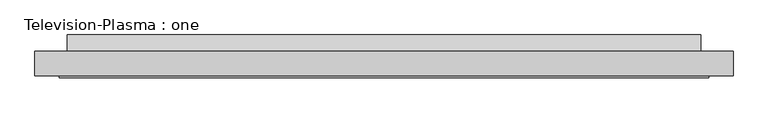
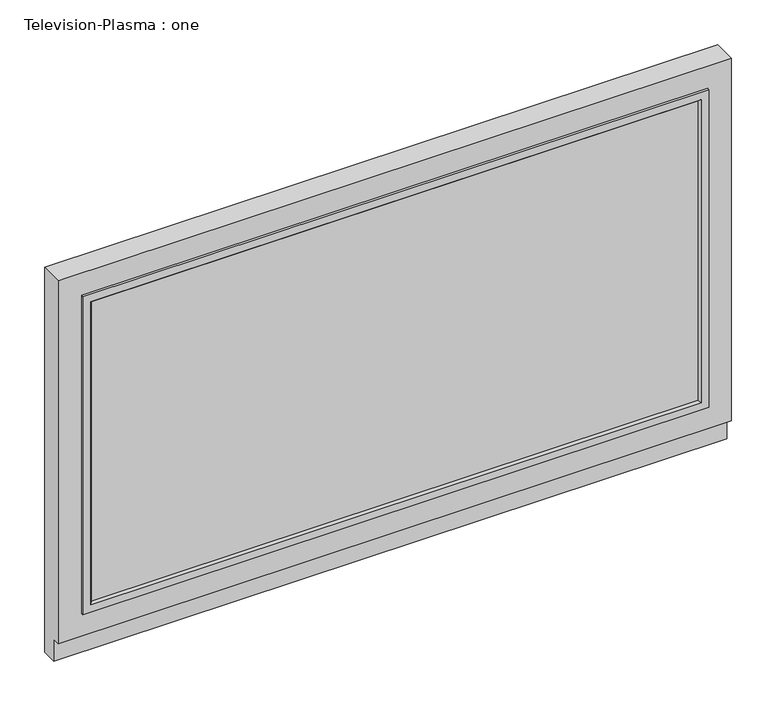
"""IFC4 building model written with IfcOpenShell, lengths in millimetres: furniture geometry, Television-Plasma : one."""

import ifcopenshell
import ifcopenshell.guid

model = None  # the IFC model being written
_history = None  # IfcOwnerHistory: only IFC2X3 demands one
_inside = {}  # id of a spatial element -> (the spatial element, [elements in it])
_under = {}  # id of a project, library or spatial element -> (it, [spatial elements below it])
_declared = {}  # id of a project -> (the project, [libraries it declares])
_typed = {}  # id of a type object -> (the type object, [elements of that type])
_made_of = {}  # id of a material, layer set ... -> (it, [elements and type objects made of it])


def new_model(schema):
    """Start an empty IFC model of exactly this schema.

    Asked for "IFC4X3", IfcOpenShell would pick the latest addendum, in which some entities
    have other attributes; the version numbers below select the first issue.
    IFC2X3 requires an IfcOwnerHistory on every rooted entity: one is made here for all.
    """
    global model, _history
    if schema == "IFC4X3":
        model = ifcopenshell.file(schema_version=(4, 3, 0, 0))
    else:
        model = ifcopenshell.file(schema=schema)
    _inside.clear()
    _under.clear()
    _declared.clear()
    _typed.clear()
    _made_of.clear()
    _history = None
    if model.schema == "IFC2X3":
        org = make("IfcOrganization", Name="unknown")
        user = make(
            "IfcPersonAndOrganization",
            ThePerson=make("IfcPerson", FamilyName="unknown"),
            TheOrganization=org,
        )
        app = make(
            "IfcApplication",
            ApplicationDeveloper=org,
            Version="unknown",
            ApplicationFullName="unknown",
            ApplicationIdentifier="unknown",
        )
        _history = make(
            "IfcOwnerHistory",
            OwningUser=user,
            OwningApplication=app,
            ChangeAction="ADDED",
            CreationDate=0,
        )
    return model


def make(cls, **values):
    """One entity of the class cls with the attributes given. An attribute that is None is left unset."""
    return model.create_entity(
        cls, **{name: value for name, value in values.items() if value is not None}
    )


def rooted(cls, **values):
    """An entity with a GlobalId (a new one), such as an element, a storey or a relation."""
    return make(cls, GlobalId=ifcopenshell.guid.new(), OwnerHistory=_history, **values)


def si_unit(unit_type, name, prefix=None):
    """IfcSIUnit, for example si_unit("LENGTHUNIT", "METRE", prefix="MILLI")."""
    return make("IfcSIUnit", UnitType=unit_type, Prefix=prefix, Name=name)


def assignment(units):
    """IfcUnitAssignment: the units of a project."""
    return None if units is None else make("IfcUnitAssignment", Units=units)


def point(xyz):
    """IfcCartesianPoint."""
    return None if xyz is None else make("IfcCartesianPoint", Coordinates=xyz)


def direction(xyz):
    """IfcDirection."""
    return None if xyz is None else make("IfcDirection", DirectionRatios=xyz)


def frame(location, z_axis=None, x_axis=None):
    """IfcAxis2Placement3D, a coordinate frame: its origin and axes. An axis left out is left unset."""
    return make(
        "IfcAxis2Placement3D",
        Location=point(location),
        Axis=direction(z_axis),
        RefDirection=direction(x_axis),
    )


def origin():
    """The frame at (0, 0, 0) with its axes left unset."""
    return frame((0.0, 0.0, 0.0))


def place(relative_to, where):
    """IfcLocalPlacement: puts the frame where relative to a parent placement (None: the world)."""
    return make(
        "IfcLocalPlacement", PlacementRelTo=relative_to, RelativePlacement=where
    )


def context(
    kind, dimensions, precision=None, world=None, true_north=None, identifier=None
):
    """IfcGeometricRepresentationContext, for example the 3D "Model" context."""
    return make(
        "IfcGeometricRepresentationContext",
        ContextIdentifier=identifier,
        ContextType=kind,
        CoordinateSpaceDimension=dimensions,
        Precision=precision,
        WorldCoordinateSystem=world,
        TrueNorth=true_north,
    )


def project(units=None, contexts=None):
    """IfcProject with its units and contexts."""
    return rooted(
        "IfcProject",
        Name="project",
        RepresentationContexts=contexts,
        UnitsInContext=assignment(units),
    )


def spatial(cls, under=None, at=None, **own):
    """A site, building, storey or space (cls), placed at a placement, below another one or the project."""
    s = rooted(cls, ObjectPlacement=at, **own)
    if under is not None:
        _under.setdefault(under.id(), (under, []))[1].append(s)
    return s


def polyline(points):
    """IfcPolyline through the points."""
    return make("IfcPolyline", Points=[point(p) for p in points])


def outline(outer, holes=None, kind="AREA"):
    """IfcArbitraryClosedProfileDef: a profile drawn as a closed curve; with holes, ...WithVoids."""
    if holes is None:
        return make("IfcArbitraryClosedProfileDef", ProfileType=kind, OuterCurve=outer)
    return make(
        "IfcArbitraryProfileDefWithVoids",
        ProfileType=kind,
        OuterCurve=outer,
        InnerCurves=holes,
    )


def extrude(swept, where, along, depth):
    """IfcExtrudedAreaSolid: the profile swept, set in the frame where, extruded along a direction by depth."""
    return make(
        "IfcExtrudedAreaSolid",
        SweptArea=swept,
        Position=where,
        ExtrudedDirection=direction(along),
        Depth=depth,
    )


def faces_of(points, faces, orient=None, outer=None):
    """IfcFace entities. A face is a list of loops; a loop is a list of indices into points, from 0.

    orient and outer hold one flag for each loop. By default every Orientation is true, the
    first loop of a face is its IfcFaceOuterBound and the others are IfcFaceBound.
    """
    made = []
    for i, loops in enumerate(faces):
        bounds = []
        for j, loop in enumerate(loops):
            is_outer = j == 0 if outer is None else outer[i][j]
            bounds.append(
                make(
                    "IfcFaceOuterBound" if is_outer else "IfcFaceBound",
                    Bound=make("IfcPolyLoop", Polygon=[points[k] for k in loop]),
                    Orientation=True if orient is None else orient[i][j],
                )
            )
        made.append(make("IfcFace", Bounds=bounds))
    return made


def faceted_brep(points, faces, orient=None, outer=None, voids=None):
    """IfcFacetedBrep: a solid bounded by flat faces; with voids (closed shells), ...WithVoids."""
    shared = [point(p) for p in points]
    hull = make("IfcClosedShell", CfsFaces=faces_of(shared, faces, orient, outer))
    if voids is None:
        return make("IfcFacetedBrep", Outer=hull)
    return make(
        "IfcFacetedBrepWithVoids",
        Outer=hull,
        Voids=[
            make(cls, CfsFaces=faces_of(shared, fs, o, b)) for cls, fs, o, b in voids
        ],
    )


def shape(context_of_items, identifier, shape_type, items):
    """IfcShapeRepresentation: the items that make up one representation, for example the "Body"."""
    return make(
        "IfcShapeRepresentation",
        ContextOfItems=context_of_items,
        RepresentationIdentifier=identifier,
        RepresentationType=shape_type,
        Items=items,
    )


def source(mapping_origin, context_of_items, identifier, shape_type, items):
    """IfcRepresentationMap: a shape defined once, which mapped items show again and again."""
    return make(
        "IfcRepresentationMap",
        MappingOrigin=mapping_origin,
        MappedRepresentation=shape(context_of_items, identifier, shape_type, items),
    )


def transform(
    local_origin,
    x_axis=None,
    y_axis=None,
    z_axis=None,
    scale=None,
    scale2=None,
    scale3=None,
    uniform=True,
):
    """IfcCartesianTransformationOperator3D, or its non-uniform kind. x_axis, y_axis, z_axis: its Axis1, 2, 3."""
    if uniform:
        return make(
            "IfcCartesianTransformationOperator3D",
            Axis1=direction(x_axis),
            Axis2=direction(y_axis),
            LocalOrigin=point(local_origin),
            Scale=scale,
            Axis3=direction(z_axis),
        )
    return make(
        "IfcCartesianTransformationOperator3DnonUniform",
        Axis1=direction(x_axis),
        Axis2=direction(y_axis),
        LocalOrigin=point(local_origin),
        Scale=scale,
        Axis3=direction(z_axis),
        Scale2=scale2,
        Scale3=scale3,
    )


def mapped(mapping_source, mapping_target):
    """IfcMappedItem: shows the shape of a source again, moved by a transform."""
    return make(
        "IfcMappedItem", MappingSource=mapping_source, MappingTarget=mapping_target
    )


def made_of(thing, what):
    """Note that an element or type object is made of a material, layer set ...; save() writes the relation."""
    if what is not None:
        _made_of.setdefault(what.id(), (what, []))[1].append(thing)
    return thing


def element(
    cls,
    number,
    at=None,
    inside=None,
    cuts=None,
    type_object=None,
    material=None,
    context=None,
    identifier="Body",
    shape_type=None,
    held_by="IfcProductDefinitionShape",
    body=None,
    shapes=None,
    **own,
):
    """One element of the class cls, such as IfcWall. Its Tag is "e" and its number.

    at: its placement. inside: the storey or other place that contains it. cuts: it is an
    opening in that element (IfcRelVoidsElement). A single representation is given by context,
    identifier, shape_type and body (its items); several are given by shapes. held_by: the class
    of the entity that holds the representations. save() writes the other relations.
    """
    e = rooted(cls, Tag="e%d" % number, ObjectPlacement=at, **own)
    if body is not None:
        shapes = [shape(context, identifier, shape_type, body)]
    if shapes is not None:
        e.Representation = make(held_by, Representations=shapes)
    if inside is not None:
        _inside.setdefault(inside.id(), (inside, []))[1].append(e)
    if cuts is not None:
        rooted(
            "IfcRelVoidsElement", RelatingBuildingElement=cuts, RelatedOpeningElement=e
        )
    if type_object is not None:
        _typed.setdefault(type_object.id(), (type_object, []))[1].append(e)
    return made_of(e, material)


def aggregate(whole, parts):
    """IfcRelAggregates: a whole, such as a stair, and the parts it consists of."""
    return rooted("IfcRelAggregates", RelatingObject=whole, RelatedObjects=parts)


def save(model, path):
    """Write the relations noted so far, then the file.

    IfcRelAggregates (storeys below a building ...), IfcRelContainedInSpatialStructure (elements
    in a storey), IfcRelDefinesByType, IfcRelAssociatesMaterial and IfcRelDeclares: one each for
    every whole, place, type object, material and project.
    """
    for whole, parts in _under.values():
        aggregate(whole, parts)
    for where, things in _inside.values():
        rooted(
            "IfcRelContainedInSpatialStructure",
            RelatedElements=things,
            RelatingStructure=where,
        )
    for kind, things in _typed.values():
        rooted("IfcRelDefinesByType", RelatedObjects=things, RelatingType=kind)
    for what, things in _made_of.values():
        rooted("IfcRelAssociatesMaterial", RelatedObjects=things, RelatingMaterial=what)
    for by, libraries in _declared.values():
        rooted("IfcRelDeclares", RelatingContext=by, RelatedDefinitions=libraries)
    model.write(path)


def television_plasma_one_caf774cc(model_context):
    return source(origin(), model_context, "Body", "SolidModel", [
        faceted_brep([(603.25, -25.4, 660.4), (-488.95, -25.4, 660.4), (-488.95, -63.5, 660.4), (603.25, -63.5, 660.4), (-488.95, -25.4, 0.0), (603.25, -25.4, 0.0), (603.25, -50.8, 0.0), (-488.95, -50.8, 0.0), (-488.95, -50.8, 38.1), (-488.95, -63.5, 38.1), (603.25, -63.5, 38.1), (565.15, -63.5, 622.3), (565.15, -63.5, 76.2), (-450.85, -63.5, 76.2), (-450.85, -63.5, 622.3), (603.25, -50.8, 38.1), (565.15, -48.7720413, 622.3), (-450.85, -48.7720413, 622.3), (-450.85, -48.7720413, 76.2), (565.15, -48.7720413, 76.2)], [[[0, 1, 2, 3]], [[4, 5, 6, 7]], [[1, 0, 5, 4]], [[2, 1, 4, 7, 8, 9]], [[3, 2, 9, 10], [11, 12, 13, 14]], [[0, 3, 10, 15, 6, 5]], [[16, 17, 18, 19]], [[16, 19, 12, 11]], [[19, 18, 13, 12]], [[18, 17, 14, 13]], [[17, 16, 11, 14]], [[15, 8, 7, 6]], [[8, 15, 10, 9]]]),
        faceted_brep([(549.275, -63.5, 92.075), (552.45, -66.675, 88.9), (552.45, -66.675, 608.80625), (549.275, -63.5, 605.63125), (552.45, -48.7720413, 88.9), (552.45, -63.5, 88.9), (552.45, -63.5, 608.80625), (552.45, -48.7720413, 608.80625), (565.15, -66.675, 76.2), (565.15, -48.7720413, 76.2), (565.15, -48.7720413, 621.50625), (565.15, -66.675, 621.50625), (-438.15, -66.675, 608.80625), (-434.975, -63.5, 605.63125), (-438.15, -63.5, 608.80625), (-438.15, -48.7720413, 608.80625), (-450.85, -48.7720413, 621.50625), (-450.85, -66.675, 621.50625), (-438.15, -66.675, 88.9), (-434.975, -63.5, 92.075), (-438.15, -63.5, 88.9), (-438.15, -48.7720413, 88.9), (-450.85, -48.7720413, 76.2), (-450.85, -66.675, 76.2)], [[[0, 1, 2, 3]], [[4, 5, 6, 7]], [[8, 9, 10, 11]], [[3, 2, 12, 13]], [[7, 6, 14, 15]], [[11, 10, 16, 17]], [[13, 12, 18, 19]], [[15, 14, 20, 21]], [[17, 16, 22, 23]], [[11, 17, 23, 8], [1, 18, 12, 2]], [[19, 18, 1, 0]], [[5, 20, 14, 6], [3, 13, 19, 0]], [[21, 20, 5, 4]], [[9, 22, 16, 10], [7, 15, 21, 4]], [[23, 22, 9, 8]]]),
        extrude(outline(polyline([(552.45, -63.5), (-438.15, -63.5), (-438.15, -48.7720413), (552.45, -48.7720413), (552.45, -63.5)])), frame((0.0, 0.0, 88.9), z_axis=(0.0, 0.0, 1.0), x_axis=(1.0, 0.0, 0.0)), (0.0, 0.0, 1.0), 520.7),
        extrude(outline(polyline([(0.0, 574.8688953), (0.0, 38.1), (-25.4, 38.1), (-25.4, 609.6), (0.0, 574.8688953)])), frame((-438.15, 0.0, 0.0), z_axis=(1.0, 0.0, 0.0), x_axis=(0.0, 1.0, 0.0)), (0.0, 0.0, 1.0), 990.6),
    ])


if __name__ == "__main__":
    model = new_model("IFC4")
    model_context = context("Model", 3, world=origin())
    ifc_project = project(units=[si_unit("LENGTHUNIT", "METRE", prefix="MILLI")], contexts=[model_context])
    site = spatial("IfcSite", under=ifc_project)
    building = spatial("IfcBuilding", under=site)
    placement = place(None, origin())
    television_plasma_one_shape = television_plasma_one_caf774cc(model_context)
    element("IfcFurniture", 1, ObjectType="Television-Plasma : one", at=placement, inside=building, context=model_context, shape_type="MappedRepresentation", body=[
        mapped(television_plasma_one_shape, transform((0.0, 0.0, 0.0), x_axis=(1.0, 0.0, 0.0), y_axis=(0.0, 1.0, 0.0), z_axis=(0.0, 0.0, 1.0))),
    ])
    save(model, "model.ifc")

# Revit data of these elements
# Type "Television-Plasma : one"
#   Assembly Code = "E2020200"
#   Depth = 0' - 2 1/2"
#   Height = 2' - 2"
#   Width = 3' - 7"
#   Cabinet Material = Plastic - Gray
# Element 1 (IfcFurniture, "Television-Plasma : one")
#   Materials on its faces: "Plastic - Black", "Plastic - Gray", "tv"
# Materials
#   "Plastic - Gray": class "Plastic", colour RGB 134 134 134, transparency 0
#   "Plastic - Black": class "Plastic", colour RGB 0 0 0, transparency 0
#   "tv": class "Glass", colour RGB 140 218 255, transparency 0, Description = "Soda Lime Glass", Cost = 0
